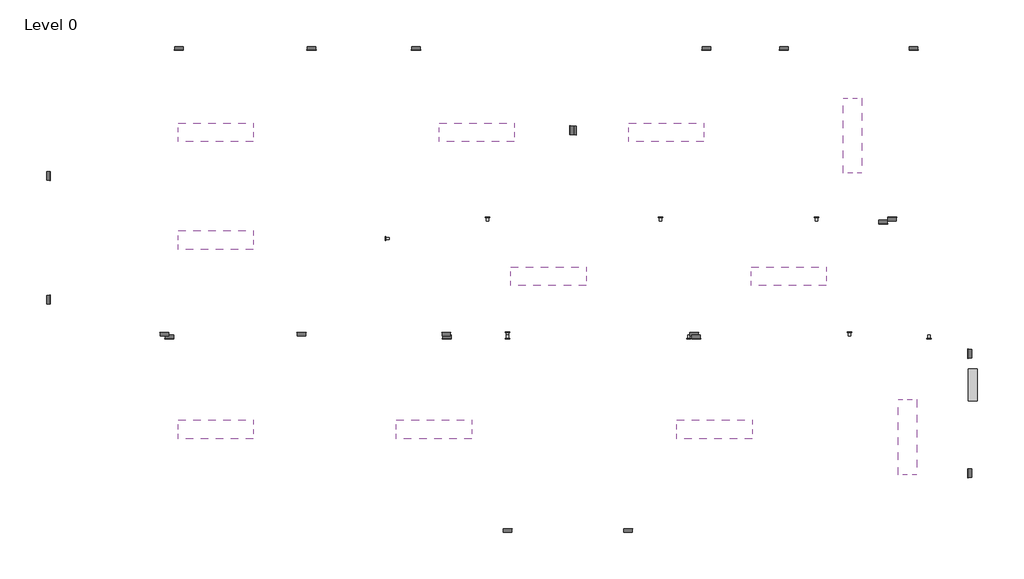
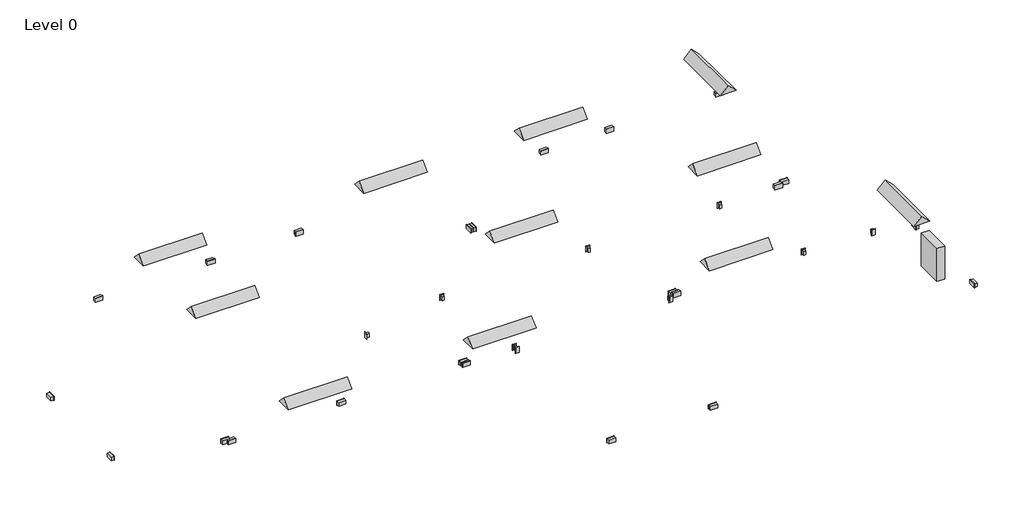
# One storey: 24 proxies, 11 light fixtures, 9 switching devices.
"""IFC4 building model written with IfcOpenShell, lengths in millimetres."""

import ifcopenshell
import ifcopenshell.guid

model = None  # the IFC model being written
_history = None  # IfcOwnerHistory: only IFC2X3 demands one
_inside = {}  # id of a spatial element -> (the spatial element, [elements in it])
_under = {}  # id of a project, library or spatial element -> (it, [spatial elements below it])
_declared = {}  # id of a project -> (the project, [libraries it declares])
_typed = {}  # id of a type object -> (the type object, [elements of that type])
_made_of = {}  # id of a material, layer set ... -> (it, [elements and type objects made of it])


def new_model(schema):
    """Start an empty IFC model of exactly this schema.

    Asked for "IFC4X3", IfcOpenShell would pick the latest addendum, in which some entities
    have other attributes; the version numbers below select the first issue.
    IFC2X3 requires an IfcOwnerHistory on every rooted entity: one is made here for all.
    """
    global model, _history
    if schema == "IFC4X3":
        model = ifcopenshell.file(schema_version=(4, 3, 0, 0))
    else:
        model = ifcopenshell.file(schema=schema)
    _inside.clear()
    _under.clear()
    _declared.clear()
    _typed.clear()
    _made_of.clear()
    _history = None
    if model.schema == "IFC2X3":
        org = make("IfcOrganization", Name="unknown")
        user = make(
            "IfcPersonAndOrganization",
            ThePerson=make("IfcPerson", FamilyName="unknown"),
            TheOrganization=org,
        )
        app = make(
            "IfcApplication",
            ApplicationDeveloper=org,
            Version="unknown",
            ApplicationFullName="unknown",
            ApplicationIdentifier="unknown",
        )
        _history = make(
            "IfcOwnerHistory",
            OwningUser=user,
            OwningApplication=app,
            ChangeAction="ADDED",
            CreationDate=0,
        )
    return model


def make(cls, **values):
    """One entity of the class cls with the attributes given. An attribute that is None is left unset."""
    return model.create_entity(
        cls, **{name: value for name, value in values.items() if value is not None}
    )


def rooted(cls, **values):
    """An entity with a GlobalId (a new one), such as an element, a storey or a relation."""
    return make(cls, GlobalId=ifcopenshell.guid.new(), OwnerHistory=_history, **values)


def si_unit(unit_type, name, prefix=None):
    """IfcSIUnit, for example si_unit("LENGTHUNIT", "METRE", prefix="MILLI")."""
    return make("IfcSIUnit", UnitType=unit_type, Prefix=prefix, Name=name)


def assignment(units):
    """IfcUnitAssignment: the units of a project."""
    return None if units is None else make("IfcUnitAssignment", Units=units)


def point(xyz):
    """IfcCartesianPoint."""
    return None if xyz is None else make("IfcCartesianPoint", Coordinates=xyz)


def direction(xyz):
    """IfcDirection."""
    return None if xyz is None else make("IfcDirection", DirectionRatios=xyz)


def frame(location, z_axis=None, x_axis=None):
    """IfcAxis2Placement3D, a coordinate frame: its origin and axes. An axis left out is left unset."""
    return make(
        "IfcAxis2Placement3D",
        Location=point(location),
        Axis=direction(z_axis),
        RefDirection=direction(x_axis),
    )


def origin():
    """The frame at (0, 0, 0) with its axes left unset."""
    return frame((0.0, 0.0, 0.0))


def origin_with_axes():
    """The frame at (0, 0, 0) with the z axis (0, 0, 1) and the x axis (1, 0, 0) written out."""
    return frame((0.0, 0.0, 0.0), z_axis=(0.0, 0.0, 1.0), x_axis=(1.0, 0.0, 0.0))


def place(relative_to, where):
    """IfcLocalPlacement: puts the frame where relative to a parent placement (None: the world)."""
    return make(
        "IfcLocalPlacement", PlacementRelTo=relative_to, RelativePlacement=where
    )


def context(
    kind, dimensions, precision=None, world=None, true_north=None, identifier=None
):
    """IfcGeometricRepresentationContext, for example the 3D "Model" context."""
    return make(
        "IfcGeometricRepresentationContext",
        ContextIdentifier=identifier,
        ContextType=kind,
        CoordinateSpaceDimension=dimensions,
        Precision=precision,
        WorldCoordinateSystem=world,
        TrueNorth=true_north,
    )


def project(units=None, contexts=None):
    """IfcProject with its units and contexts."""
    return rooted(
        "IfcProject",
        Name="project",
        RepresentationContexts=contexts,
        UnitsInContext=assignment(units),
    )


def spatial(cls, under=None, at=None, **own):
    """A site, building, storey or space (cls), placed at a placement, below another one or the project."""
    s = rooted(cls, ObjectPlacement=at, **own)
    if under is not None:
        _under.setdefault(under.id(), (under, []))[1].append(s)
    return s


def polyline(points):
    """IfcPolyline through the points."""
    return make("IfcPolyline", Points=[point(p) for p in points])


def outline(outer, holes=None, kind="AREA"):
    """IfcArbitraryClosedProfileDef: a profile drawn as a closed curve; with holes, ...WithVoids."""
    if holes is None:
        return make("IfcArbitraryClosedProfileDef", ProfileType=kind, OuterCurve=outer)
    return make(
        "IfcArbitraryProfileDefWithVoids",
        ProfileType=kind,
        OuterCurve=outer,
        InnerCurves=holes,
    )


def extrude(swept, where, along, depth):
    """IfcExtrudedAreaSolid: the profile swept, set in the frame where, extruded along a direction by depth."""
    return make(
        "IfcExtrudedAreaSolid",
        SweptArea=swept,
        Position=where,
        ExtrudedDirection=direction(along),
        Depth=depth,
    )


def shape(context_of_items, identifier, shape_type, items):
    """IfcShapeRepresentation: the items that make up one representation, for example the "Body"."""
    return make(
        "IfcShapeRepresentation",
        ContextOfItems=context_of_items,
        RepresentationIdentifier=identifier,
        RepresentationType=shape_type,
        Items=items,
    )


def source(mapping_origin, context_of_items, identifier, shape_type, items):
    """IfcRepresentationMap: a shape defined once, which mapped items show again and again."""
    return make(
        "IfcRepresentationMap",
        MappingOrigin=mapping_origin,
        MappedRepresentation=shape(context_of_items, identifier, shape_type, items),
    )


def transform(
    local_origin,
    x_axis=None,
    y_axis=None,
    z_axis=None,
    scale=None,
    scale2=None,
    scale3=None,
    uniform=True,
):
    """IfcCartesianTransformationOperator3D, or its non-uniform kind. x_axis, y_axis, z_axis: its Axis1, 2, 3."""
    if uniform:
        return make(
            "IfcCartesianTransformationOperator3D",
            Axis1=direction(x_axis),
            Axis2=direction(y_axis),
            LocalOrigin=point(local_origin),
            Scale=scale,
            Axis3=direction(z_axis),
        )
    return make(
        "IfcCartesianTransformationOperator3DnonUniform",
        Axis1=direction(x_axis),
        Axis2=direction(y_axis),
        LocalOrigin=point(local_origin),
        Scale=scale,
        Axis3=direction(z_axis),
        Scale2=scale2,
        Scale3=scale3,
    )


def mapped(mapping_source, mapping_target):
    """IfcMappedItem: shows the shape of a source again, moved by a transform."""
    return make(
        "IfcMappedItem", MappingSource=mapping_source, MappingTarget=mapping_target
    )


def made_of(thing, what):
    """Note that an element or type object is made of a material, layer set ...; save() writes the relation."""
    if what is not None:
        _made_of.setdefault(what.id(), (what, []))[1].append(thing)
    return thing


def element(
    cls,
    number,
    at=None,
    inside=None,
    cuts=None,
    type_object=None,
    material=None,
    context=None,
    identifier="Body",
    shape_type=None,
    held_by="IfcProductDefinitionShape",
    body=None,
    shapes=None,
    **own,
):
    """One element of the class cls, such as IfcWall. Its Tag is "e" and its number.

    at: its placement. inside: the storey or other place that contains it. cuts: it is an
    opening in that element (IfcRelVoidsElement). A single representation is given by context,
    identifier, shape_type and body (its items); several are given by shapes. held_by: the class
    of the entity that holds the representations. save() writes the other relations.
    """
    e = rooted(cls, Tag="e%d" % number, ObjectPlacement=at, **own)
    if body is not None:
        shapes = [shape(context, identifier, shape_type, body)]
    if shapes is not None:
        e.Representation = make(held_by, Representations=shapes)
    if inside is not None:
        _inside.setdefault(inside.id(), (inside, []))[1].append(e)
    if cuts is not None:
        rooted(
            "IfcRelVoidsElement", RelatingBuildingElement=cuts, RelatedOpeningElement=e
        )
    if type_object is not None:
        _typed.setdefault(type_object.id(), (type_object, []))[1].append(e)
    return made_of(e, material)


def aggregate(whole, parts):
    """IfcRelAggregates: a whole, such as a stair, and the parts it consists of."""
    return rooted("IfcRelAggregates", RelatingObject=whole, RelatedObjects=parts)


def save(model, path):
    """Write the relations noted so far, then the file.

    IfcRelAggregates (storeys below a building ...), IfcRelContainedInSpatialStructure (elements
    in a storey), IfcRelDefinesByType, IfcRelAssociatesMaterial and IfcRelDeclares: one each for
    every whole, place, type object, material and project.
    """
    for whole, parts in _under.values():
        aggregate(whole, parts)
    for where, things in _inside.values():
        rooted(
            "IfcRelContainedInSpatialStructure",
            RelatedElements=things,
            RelatingStructure=where,
        )
    for kind, things in _typed.values():
        rooted("IfcRelDefinesByType", RelatedObjects=things, RelatingType=kind)
    for what, things in _made_of.values():
        rooted("IfcRelAssociatesMaterial", RelatedObjects=things, RelatingMaterial=what)
    for by, libraries in _declared.values():
        rooted("IfcRelDeclares", RelatingContext=by, RelatedDefinitions=libraries)
    model.write(path)


def lighting_and_appliance_panelboard_400v_mlo_125_a_11cb7106(model_context):
    return source(origin(), model_context, "Body", "SweptSolid", [
        extrude(outline(polyline([(254.0, -660.4), (-254.0, -660.4), (-254.0, 0.0), (254.0, 0.0), (254.0, -660.4)])), frame((0.0, 0.0, -146.1), z_axis=(0.0, 0.0, 1.0), x_axis=(1.0, 0.0, 0.0)), (0.0, 0.0, 1.0), 146.1),
    ])


def twin_switched_socket_outlet_standard_0deee84c(model_context):
    return source(origin(), model_context, "Body", "SweptSolid", [
        extrude(outline(polyline([(67.5, 37.5), (67.5, -37.5), (-67.5, -37.5), (-67.5, 37.5), (67.5, 37.5)])), frame((0.0, 0.0, -53.975), z_axis=(0.0, 0.0, 1.0), x_axis=(1.0, 0.0, 0.0)), (0.0, 0.0, 1.0), 53.975),
        extrude(outline(polyline([(72.5, 42.5), (72.5, -42.5), (-72.5, -42.5), (-72.5, 42.5), (72.5, 42.5)])), origin_with_axes(), (0.0, 0.0, 1.0), 4.7625),
    ])


def plain_recessed_lighting_fixture_300x1200_230_e46e8774(model_context):
    return source(origin(), model_context, "Body", "SweptSolid", [
        extrude(outline(polyline([(-300.0, 0.0), (0.0, 0.0), (-150.0, -150.0), (-300.0, 0.0)])), frame((0.0, 0.0, 0.0), z_axis=(1.0, 0.0, 0.0), x_axis=(0.0, 1.0, 0.0)), (0.0, 0.0, 1.0), 1200.0),
    ])


def lighting_switches_one_way_switch_9cbd35ee(model_context):
    return source(origin(), model_context, "Body", "SweptSolid", [
        extrude(outline(polyline([(35.0, -114.0), (-35.0, -114.0), (-35.0, 0.0), (35.0, 0.0), (35.0, -114.0)])), origin_with_axes(), (0.0, 0.0, 1.0), 5.0),
        extrude(outline(polyline([(19.0, -95.0), (-19.0, -95.0), (-19.0, -19.0), (19.0, -19.0), (19.0, -95.0)])), frame((0.0, 0.0, -54.0), z_axis=(0.0, 0.0, 1.0), x_axis=(1.0, 0.0, 0.0)), (0.0, 0.0, 1.0), 54.0),
    ])


model = new_model("IFC4")

# Units and contexts
model_context = context("Model", 3, world=origin())
ifc_project = project(units=[si_unit("LENGTHUNIT", "METRE", prefix="MILLI")], contexts=[model_context])

# Site, building, storey
site = spatial("IfcSite", under=ifc_project)
building = spatial("IfcBuilding", under=site)
storey = spatial("IfcBuildingStorey", under=building, Name="Level 0", Elevation=0.0)

# Proxies
placement = place(None, origin())
lighting_and_appliance_panelboard_400v_mlo_125_a_shape = lighting_and_appliance_panelboard_400v_mlo_125_a_11cb7106(model_context)
element("IfcBuildingElementProxy", 1, Name="Lighting and Appliance Panelboard - 400V MLO : 125 A", ObjectType="Lighting and Appliance Panelboard - 400V MLO : 125 A", at=placement, inside=storey, context=model_context, shape_type="MappedRepresentation", body=[
    mapped(lighting_and_appliance_panelboard_400v_mlo_125_a_shape, transform((7333.0126521, -1228.5996446, 1200.0), x_axis=(0.0, -1.0, 0.0), y_axis=(0.0, 0.0, 1.0), z_axis=(-1.0, 0.0, 0.0))),
])
twin_switched_socket_outlet_standard_shape = twin_switched_socket_outlet_standard_0deee84c(model_context)
element("IfcBuildingElementProxy", 2, Name="Twin Switched Socket Outlet : Standard", ObjectType="Twin Switched Socket Outlet : Standard", at=placement, inside=storey, context=model_context, shape_type="MappedRepresentation", body=[
    mapped(twin_switched_socket_outlet_standard_shape, transform((7333.0126521, -731.9030192, 1200.0), x_axis=(0.0, -1.0, 0.0), y_axis=(0.0, 0.0, 1.0), z_axis=(-1.0, 0.0, 0.0))),
])
element("IfcBuildingElementProxy", 3, Name="Twin Switched Socket Outlet : Standard", ObjectType="Twin Switched Socket Outlet : Standard", at=placement, inside=storey, context=model_context, shape_type="MappedRepresentation", body=[
    mapped(twin_switched_socket_outlet_standard_shape, transform((7333.0126521, -2640.7763248, 1200.0), x_axis=(0.0, -1.0, 0.0), y_axis=(0.0, 0.0, 1.0), z_axis=(-1.0, 0.0, 0.0))),
])
element("IfcBuildingElementProxy", 4, Name="Twin Switched Socket Outlet : Standard", ObjectType="Twin Switched Socket Outlet : Standard", at=placement, inside=storey, context=model_context, shape_type="MappedRepresentation", body=[
    mapped(twin_switched_socket_outlet_standard_shape, transform((1908.0707872, -3530.9314954, 1200.0), x_axis=(-1.0, 0.0, 0.0), y_axis=(0.0, 0.0, 1.0), z_axis=(0.0, 1.0, 0.0))),
])
element("IfcBuildingElementProxy", 5, Name="Twin Switched Socket Outlet : Standard", ObjectType="Twin Switched Socket Outlet : Standard", at=placement, inside=storey, context=model_context, shape_type="MappedRepresentation", body=[
    mapped(twin_switched_socket_outlet_standard_shape, transform((2992.0804727, -488.4314954, 1200.0), x_axis=(1.0, 0.0, 0.0), y_axis=(0.0, 0.0, 1.0), z_axis=(0.0, -1.0, 0.0))),
])
element("IfcBuildingElementProxy", 6, Name="Twin Switched Socket Outlet : Standard", ObjectType="Twin Switched Socket Outlet : Standard", at=placement, inside=storey, context=model_context, shape_type="MappedRepresentation", body=[
    mapped(twin_switched_socket_outlet_standard_shape, transform((2958.20517, -393.4314954, 1200.0), x_axis=(-1.0, 0.0, 0.0), y_axis=(0.0, 0.0, 1.0), z_axis=(0.0, 1.0, 0.0))),
])
element("IfcBuildingElementProxy", 7, Name="Twin Switched Socket Outlet : Standard", ObjectType="Twin Switched Socket Outlet : Standard", at=placement, inside=storey, context=model_context, shape_type="MappedRepresentation", body=[
    mapped(twin_switched_socket_outlet_standard_shape, transform((-14.3526395, -3530.9314954, 1200.0), x_axis=(-1.0, 0.0, 0.0), y_axis=(0.0, 0.0, 1.0), z_axis=(0.0, 1.0, 0.0))),
])
element("IfcBuildingElementProxy", 8, Name="Twin Switched Socket Outlet : Standard", ObjectType="Twin Switched Socket Outlet : Standard", at=placement, inside=storey, context=model_context, shape_type="MappedRepresentation", body=[
    mapped(twin_switched_socket_outlet_standard_shape, transform((4391.3814995, 4119.0685046, 1200.0), x_axis=(1.0, 0.0, 0.0), y_axis=(0.0, 0.0, 1.0), z_axis=(0.0, -1.0, 0.0))),
])
element("IfcBuildingElementProxy", 9, Name="Twin Switched Socket Outlet : Standard", ObjectType="Twin Switched Socket Outlet : Standard", at=placement, inside=storey, context=model_context, shape_type="MappedRepresentation", body=[
    mapped(twin_switched_socket_outlet_standard_shape, transform((6460.720641, 4119.0685046, 1200.0), x_axis=(1.0, 0.0, 0.0), y_axis=(0.0, 0.0, 1.0), z_axis=(0.0, -1.0, 0.0))),
])
element("IfcBuildingElementProxy", 10, Name="Twin Switched Socket Outlet : Standard", ObjectType="Twin Switched Socket Outlet : Standard", at=placement, inside=storey, context=model_context, shape_type="MappedRepresentation", body=[
    mapped(twin_switched_socket_outlet_standard_shape, transform((3154.1965323, 4119.0685046, 1200.0), x_axis=(1.0, 0.0, 0.0), y_axis=(0.0, 0.0, 1.0), z_axis=(0.0, -1.0, 0.0))),
])
element("IfcBuildingElementProxy", 11, Name="Twin Switched Socket Outlet : Standard", ObjectType="Twin Switched Socket Outlet : Standard", at=placement, inside=storey, context=model_context, shape_type="MappedRepresentation", body=[
    mapped(twin_switched_socket_outlet_standard_shape, transform((-1477.8828984, 4119.0685046, 1200.0), x_axis=(1.0, 0.0, 0.0), y_axis=(0.0, 0.0, 1.0), z_axis=(0.0, -1.0, 0.0))),
])
element("IfcBuildingElementProxy", 12, Name="Twin Switched Socket Outlet : Standard", ObjectType="Twin Switched Socket Outlet : Standard", at=placement, inside=storey, context=model_context, shape_type="MappedRepresentation", body=[
    mapped(twin_switched_socket_outlet_standard_shape, transform((-994.5789843, -393.4314954, 1200.0), x_axis=(-1.0, 0.0, 0.0), y_axis=(0.0, 0.0, 1.0), z_axis=(0.0, 1.0, 0.0))),
])
element("IfcBuildingElementProxy", 13, Name="Twin Switched Socket Outlet : Standard", ObjectType="Twin Switched Socket Outlet : Standard", at=placement, inside=storey, context=model_context, shape_type="MappedRepresentation", body=[
    mapped(twin_switched_socket_outlet_standard_shape, transform((-983.8752261, -488.4314954, 1200.0), x_axis=(1.0, 0.0, 0.0), y_axis=(0.0, 0.0, 1.0), z_axis=(0.0, -1.0, 0.0))),
])
element("IfcBuildingElementProxy", 14, Name="Twin Switched Socket Outlet : Standard", ObjectType="Twin Switched Socket Outlet : Standard", at=placement, inside=storey, context=model_context, shape_type="MappedRepresentation", body=[
    mapped(twin_switched_socket_outlet_standard_shape, transform((-7316.9873479, 2106.2473929, 1200.0), x_axis=(0.0, 1.0, 0.0), y_axis=(0.0, 0.0, 1.0), z_axis=(1.0, 0.0, 0.0))),
])
element("IfcBuildingElementProxy", 15, Name="Twin Switched Socket Outlet : Standard", ObjectType="Twin Switched Socket Outlet : Standard", at=placement, inside=storey, context=model_context, shape_type="MappedRepresentation", body=[
    mapped(twin_switched_socket_outlet_standard_shape, transform((-7316.9873479, 133.0110122, 1200.0), x_axis=(0.0, 1.0, 0.0), y_axis=(0.0, 0.0, 1.0), z_axis=(1.0, 0.0, 0.0))),
])
element("IfcBuildingElementProxy", 16, Name="Twin Switched Socket Outlet : Standard", ObjectType="Twin Switched Socket Outlet : Standard", at=placement, inside=storey, context=model_context, shape_type="MappedRepresentation", body=[
    mapped(twin_switched_socket_outlet_standard_shape, transform((-5491.7999145, -393.4314954, 1200.0), x_axis=(-1.0, 0.0, 0.0), y_axis=(0.0, 0.0, 1.0), z_axis=(0.0, 1.0, 0.0))),
])
element("IfcBuildingElementProxy", 17, Name="Twin Switched Socket Outlet : Standard", ObjectType="Twin Switched Socket Outlet : Standard", at=placement, inside=storey, context=model_context, shape_type="MappedRepresentation", body=[
    mapped(twin_switched_socket_outlet_standard_shape, transform((-5410.6999104, -488.4314954, 1200.0), x_axis=(1.0, 0.0, 0.0), y_axis=(0.0, 0.0, 1.0), z_axis=(0.0, -1.0, 0.0))),
])
element("IfcBuildingElementProxy", 18, Name="Twin Switched Socket Outlet : Standard", ObjectType="Twin Switched Socket Outlet : Standard", at=placement, inside=storey, context=model_context, shape_type="MappedRepresentation", body=[
    mapped(twin_switched_socket_outlet_standard_shape, transform((-5260.1397144, 4119.0685046, 1200.0), x_axis=(1.0, 0.0, 0.0), y_axis=(0.0, 0.0, 1.0), z_axis=(0.0, -1.0, 0.0))),
])
element("IfcBuildingElementProxy", 19, Name="Twin Switched Socket Outlet : Standard", ObjectType="Twin Switched Socket Outlet : Standard", at=placement, inside=storey, context=model_context, shape_type="MappedRepresentation", body=[
    mapped(twin_switched_socket_outlet_standard_shape, transform((-3144.1513827, 4119.0685046, 1200.0), x_axis=(1.0, 0.0, 0.0), y_axis=(0.0, 0.0, 1.0), z_axis=(0.0, -1.0, 0.0))),
])
element("IfcBuildingElementProxy", 20, Name="Twin Switched Socket Outlet : Standard", ObjectType="Twin Switched Socket Outlet : Standard", at=placement, inside=storey, context=model_context, shape_type="MappedRepresentation", body=[
    mapped(twin_switched_socket_outlet_standard_shape, transform((-3304.0957389, -393.4314954, 1200.0), x_axis=(-1.0, 0.0, 0.0), y_axis=(0.0, 0.0, 1.0), z_axis=(0.0, 1.0, 0.0))),
])
element("IfcBuildingElementProxy", 21, Name="Twin Switched Socket Outlet : Standard", ObjectType="Twin Switched Socket Outlet : Standard", at=placement, inside=storey, context=model_context, shape_type="MappedRepresentation", body=[
    mapped(twin_switched_socket_outlet_standard_shape, transform((983.0126521, 2835.1015679, 1200.0), x_axis=(0.0, -1.0, 0.0), y_axis=(0.0, 0.0, 1.0), z_axis=(-1.0, 0.0, 0.0))),
])
element("IfcBuildingElementProxy", 22, Name="Twin Switched Socket Outlet : Standard", ObjectType="Twin Switched Socket Outlet : Standard", at=placement, inside=storey, context=model_context, shape_type="MappedRepresentation", body=[
    mapped(twin_switched_socket_outlet_standard_shape, transform((1078.0126521, 2831.4402609, 1200.0), x_axis=(0.0, 1.0, 0.0), y_axis=(0.0, 0.0, 1.0), z_axis=(1.0, 0.0, 0.0))),
])
element("IfcBuildingElementProxy", 23, Name="Twin Switched Socket Outlet : Standard", ObjectType="Twin Switched Socket Outlet : Standard", at=placement, inside=storey, context=model_context, shape_type="MappedRepresentation", body=[
    mapped(twin_switched_socket_outlet_standard_shape, transform((5974.113816, 1346.5685046, 1200.0), x_axis=(1.0, 0.0, 0.0), y_axis=(0.0, 0.0, 1.0), z_axis=(0.0, -1.0, 0.0))),
])
element("IfcBuildingElementProxy", 24, Name="Twin Switched Socket Outlet : Standard", ObjectType="Twin Switched Socket Outlet : Standard", at=placement, inside=storey, context=model_context, shape_type="MappedRepresentation", body=[
    mapped(twin_switched_socket_outlet_standard_shape, transform((6119.3761729, 1441.5685046, 1200.0), x_axis=(-1.0, 0.0, 0.0), y_axis=(0.0, 0.0, 1.0), z_axis=(0.0, 1.0, 0.0))),
])

# Light fixtures
plain_recessed_lighting_fixture_300x1200_230_shape = plain_recessed_lighting_fixture_300x1200_230_e46e8774(model_context)
element("IfcLightFixture", 25, ObjectType="Plain Recessed Lighting Fixture : 300x1200 - 230", at=placement, inside=storey, context=model_context, shape_type="MappedRepresentation", body=[
    mapped(plain_recessed_lighting_fixture_300x1200_230_shape, transform((-5270.0307392, 2652.1798309, 2750.0), x_axis=(1.0, 0.0, 0.0), y_axis=(0.0, -1.0, 0.0), z_axis=(0.0, 0.0, -1.0))),
])
element("IfcLightFixture", 26, ObjectType="Plain Recessed Lighting Fixture : 300x1200 - 230", at=placement, inside=storey, context=model_context, shape_type="MappedRepresentation", body=[
    mapped(plain_recessed_lighting_fixture_300x1200_230_shape, transform((-5270.0307392, 932.4806964, 2750.0), x_axis=(1.0, 0.0, 0.0), y_axis=(0.0, -1.0, 0.0), z_axis=(0.0, 0.0, -1.0))),
])
element("IfcLightFixture", 27, ObjectType="Plain Recessed Lighting Fixture : 300x1200 - 230", at=placement, inside=storey, context=model_context, shape_type="MappedRepresentation", body=[
    mapped(plain_recessed_lighting_fixture_300x1200_230_shape, transform((-5270.0307392, -2089.1732245, 2750.0), x_axis=(1.0, 0.0, 0.0), y_axis=(0.0, -1.0, 0.0), z_axis=(0.0, 0.0, -1.0))),
])
element("IfcLightFixture", 28, ObjectType="Plain Recessed Lighting Fixture : 300x1200 - 230", at=placement, inside=storey, context=model_context, shape_type="MappedRepresentation", body=[
    mapped(plain_recessed_lighting_fixture_300x1200_230_shape, transform((-1789.2039186, -2089.1732245, 2750.0), x_axis=(1.0, 0.0, 0.0), y_axis=(0.0, -1.0, 0.0), z_axis=(0.0, 0.0, -1.0))),
])
element("IfcLightFixture", 29, ObjectType="Plain Recessed Lighting Fixture : 300x1200 - 230", at=placement, inside=storey, context=model_context, shape_type="MappedRepresentation", body=[
    mapped(plain_recessed_lighting_fixture_300x1200_230_shape, transform((2684.0288466, -2089.1732245, 2750.0), x_axis=(1.0, 0.0, 0.0), y_axis=(0.0, -1.0, 0.0), z_axis=(0.0, 0.0, -1.0))),
])
element("IfcLightFixture", 30, ObjectType="Plain Recessed Lighting Fixture : 300x1200 - 230", at=placement, inside=storey, context=model_context, shape_type="MappedRepresentation", body=[
    mapped(plain_recessed_lighting_fixture_300x1200_230_shape, transform((-1107.8505835, 2652.1798309, 2750.0), x_axis=(1.0, 0.0, 0.0), y_axis=(0.0, -1.0, 0.0), z_axis=(0.0, 0.0, -1.0))),
])
element("IfcLightFixture", 31, ObjectType="Plain Recessed Lighting Fixture : 300x1200 - 230", at=placement, inside=storey, context=model_context, shape_type="MappedRepresentation", body=[
    mapped(plain_recessed_lighting_fixture_300x1200_230_shape, transform((1913.8033373, 2652.1798309, 2750.0), x_axis=(1.0, 0.0, 0.0), y_axis=(0.0, -1.0, 0.0), z_axis=(0.0, 0.0, -1.0))),
])
element("IfcLightFixture", 32, ObjectType="Plain Recessed Lighting Fixture : 300x1200 - 230", at=placement, inside=storey, context=model_context, shape_type="MappedRepresentation", body=[
    mapped(plain_recessed_lighting_fixture_300x1200_230_shape, transform((5336.1226433, 3350.5669994, 2750.0), x_axis=(0.0, -1.0, 0.0), y_axis=(-1.0, 0.0, 0.0), z_axis=(0.0, 0.0, -1.0))),
])
element("IfcLightFixture", 33, ObjectType="Plain Recessed Lighting Fixture : 300x1200 - 230", at=placement, inside=storey, context=model_context, shape_type="MappedRepresentation", body=[
    mapped(plain_recessed_lighting_fixture_300x1200_230_shape, transform((35.7584033, 354.8115644, 2750.0), x_axis=(1.0, 0.0, 0.0), y_axis=(0.0, -1.0, 0.0), z_axis=(0.0, 0.0, -1.0))),
])
element("IfcLightFixture", 34, ObjectType="Plain Recessed Lighting Fixture : 300x1200 - 230", at=placement, inside=storey, context=model_context, shape_type="MappedRepresentation", body=[
    mapped(plain_recessed_lighting_fixture_300x1200_230_shape, transform((3868.9911685, 354.8115644, 2750.0), x_axis=(1.0, 0.0, 0.0), y_axis=(0.0, -1.0, 0.0), z_axis=(0.0, 0.0, -1.0))),
])
element("IfcLightFixture", 35, ObjectType="Plain Recessed Lighting Fixture : 300x1200 - 230", at=placement, inside=storey, context=model_context, shape_type="MappedRepresentation", body=[
    mapped(plain_recessed_lighting_fixture_300x1200_230_shape, transform((6212.25416, -1465.5868026, 2750.0), x_axis=(0.0, -1.0, 0.0), y_axis=(-1.0, 0.0, 0.0), z_axis=(0.0, 0.0, -1.0))),
])

# Switching devices
lighting_switches_one_way_switch_shape = lighting_switches_one_way_switch_9cbd35ee(model_context)
element("IfcSwitchingDevice", 36, ObjectType="Lighting Switches : One Way Switch", at=placement, inside=storey, context=model_context, shape_type="MappedRepresentation", body=[
    mapped(lighting_switches_one_way_switch_shape, transform((-1959.4873479, 1106.2790704, 1200.0), x_axis=(0.0, -1.0, 0.0), y_axis=(0.0, 0.0, 1.0), z_axis=(-1.0, 0.0, 0.0))),
])
element("IfcSwitchingDevice", 37, ObjectType="Lighting Switches : One Way Switch", at=placement, inside=storey, context=model_context, shape_type="MappedRepresentation", body=[
    mapped(lighting_switches_one_way_switch_shape, transform((-334.0931611, 1441.5685046, 1200.0), x_axis=(-1.0, 0.0, 0.0), y_axis=(0.0, 0.0, 1.0), z_axis=(0.0, 1.0, 0.0))),
])
element("IfcSwitchingDevice", 38, ObjectType="Lighting Switches : One Way Switch", at=placement, inside=storey, context=model_context, shape_type="MappedRepresentation", body=[
    mapped(lighting_switches_one_way_switch_shape, transform((2425.9086107, 1441.5685046, 1200.0), x_axis=(-1.0, 0.0, 0.0), y_axis=(0.0, 0.0, 1.0), z_axis=(0.0, 1.0, 0.0))),
])
element("IfcSwitchingDevice", 39, ObjectType="Lighting Switches : One Way Switch", at=placement, inside=storey, context=model_context, shape_type="MappedRepresentation", body=[
    mapped(lighting_switches_one_way_switch_shape, transform((4910.5243833, 1441.5685046, 1200.0), x_axis=(-1.0, 0.0, 0.0), y_axis=(0.0, 0.0, 1.0), z_axis=(0.0, 1.0, 0.0))),
])
element("IfcSwitchingDevice", 40, ObjectType="Lighting Switches : One Way Switch", at=placement, inside=storey, context=model_context, shape_type="MappedRepresentation", body=[
    mapped(lighting_switches_one_way_switch_shape, transform((6703.5460749, -488.4314954, 1200.0), x_axis=(1.0, 0.0, 0.0), y_axis=(0.0, 0.0, 1.0), z_axis=(0.0, -1.0, 0.0))),
])
element("IfcSwitchingDevice", 41, ObjectType="Lighting Switches : One Way Switch", at=placement, inside=storey, context=model_context, shape_type="MappedRepresentation", body=[
    mapped(lighting_switches_one_way_switch_shape, transform((2874.1640336, -488.4314954, 1200.0), x_axis=(1.0, 0.0, 0.0), y_axis=(0.0, 0.0, 1.0), z_axis=(0.0, -1.0, 0.0))),
])
element("IfcSwitchingDevice", 42, ObjectType="Lighting Switches : One Way Switch", at=placement, inside=storey, context=model_context, shape_type="MappedRepresentation", body=[
    mapped(lighting_switches_one_way_switch_shape, transform((-20.2852685, -488.4314954, 1200.0), x_axis=(1.0, 0.0, 0.0), y_axis=(0.0, 0.0, 1.0), z_axis=(0.0, -1.0, 0.0))),
])
element("IfcSwitchingDevice", 43, ObjectType="Lighting Switches : Two Way Switch", at=placement, inside=storey, context=model_context, shape_type="MappedRepresentation", body=[
    mapped(lighting_switches_one_way_switch_shape, transform((-18.1392133, -393.4314954, 1200.0), x_axis=(-1.0, 0.0, 0.0), y_axis=(0.0, 0.0, 1.0), z_axis=(0.0, 1.0, 0.0))),
])
element("IfcSwitchingDevice", 44, ObjectType="Lighting Switches : Two Way Switch", at=placement, inside=storey, context=model_context, shape_type="MappedRepresentation", body=[
    mapped(lighting_switches_one_way_switch_shape, transform((5435.784517, -393.4314954, 1200.0), x_axis=(-1.0, 0.0, 0.0), y_axis=(0.0, 0.0, 1.0), z_axis=(0.0, 1.0, 0.0))),
])

save(model, "model.ifc")

# Revit data of these elements
# Project information
#   Project Issue Date = "Oct 2020"
#   Project Status = "Project Status"
#   Client Name = "Your Name Here"
#   Project Address = "Enter address here"
#   Project Name = "Revit MEP 01"
#   Project Number = "RMEP01"
# Type "Lighting and Appliance Panelboard - 400V MLO : 125 A"
#   built-in parameter 1140081 [instance default] = "Recessed"
#   built-in parameter 1140083 [instance default] = "Type 1"
#   Width = 508 mm
#   built-in parameter 1140082 [instance default] = 100 (stored number, unit not read)
#   built-in parameter 1140140 [instance default] = 1 (stored number, unit not read)
#   Height [instance default] = 660.4 mm
#   Depth = 146.1 mm
#   Default Elevation = 1200 mm
#   42 Circuit Height = 1117.6 mm
#   30 Circuit Height = 965.2 mm
#   18 Circuit Height = 660.4 mm
#   12 Circuit Height = 660.4 mm
#   built-in parameter 1140142 [instance default] = -1
#   built-in parameter 1140079 [instance default] = 12
#   built-in parameter 1155100 [instance default] = -1
#   Load Classification = Other
#   built-in parameter 1140087 [instance default] = element -7000014
# Type "Twin Switched Socket Outlet : Standard"
#   Label = "2"
#   Switch Voltage = 230 V
#   Load = 180 VA
#   Default Elevation = 1200 mm
#   Load Classification = Socket
#   Assembly Code = ""
# Type "Plain Recessed Lighting Fixture : 300x1200 - 230"
#   Photometric Web File = "1x42A12.ies"
#   Width = 300 mm
#   Wattage = 64 W
#   built-in parameter 1150110 = 1 (stored number, unit not read)
#   built-in parameter 1150109 = 1 (stored number, unit not read)
#   built-in parameter 1150113 = 1 (stored number, unit not read)
#   Tilt Angle = -90.00°
#   Lumens = 5699.84 lm
#   built-in parameter 1114217 = 0.88 (stored number, unit not read)
#   built-in parameter 1150115 = 1 (stored number, unit not read)
#   built-in parameter 1150105 = 453.579 (stored number, unit not read)
#   Length = 1200 mm
#   built-in parameter 1150112 = 1 (stored number, unit not read)
#   built-in parameter 1150114 = 1 (stored number, unit not read)
#   built-in parameter 1150107 = 4230 (stored number, unit not read)
#   built-in parameter 1150106 = 4.53579 (stored number, unit not read)
#   Emit from Rectangle Width = 300 mm
#   Emit from Rectangle Length = 1200 mm
#   built-in parameter 1150104 = 8.27394 (stored number, unit not read)
#   Depth = 150 mm
#   Default Elevation = 2000 mm
#   Ballast Voltage = 230 V
#   built-in parameter 1114218 = 0.88 (stored number, unit not read)
#   built-in parameter 1150133 = 10 (stored number, unit not read)
#   Apparent Load = 64 VA
#   built-in parameter 1150134 = 8
#   built-in parameter 1150137 = 1
#   Color Filter = 16777215
#   built-in parameter 1140040 [instance default] = 1
#   Load Classification = Lighting - Dwelling Unit
#   Emit Shape Visible in Rendering = no
#   Dimming Lamp Color Temperature Shift = (empty or 0)
#   Assembly Code = ""
# Type "Lighting Switches : One Way Switch"
#   Label = ""
#   Width = 70 mm
#   Switch Voltage [instance default] = 230 V
#   Length = 114 mm
#   Height = 59 mm
#   Default Elevation = 1200 mm
#   Apparent Load = 0 VA
#   Visibility 7 = no
#   Visibility 6 = no
#   Visibility 5 = yes
#   Visibility 4 = no
#   Visibility 3 = no
#   Visibility 2 = no
#   Visibility 1 = no
#   Number of Poles = 1
#   Load Classification = Other
# Type "Lighting Switches : Two Way Switch"
#   Label = "2"
#   Width = 70 mm
#   Switch Voltage [instance default] = 230 V
#   Length = 114 mm
#   Height = 59 mm
#   Default Elevation = 1200 mm
#   Apparent Load = 0 VA
#   Visibility 7 = no
#   Visibility 6 = no
#   Visibility 5 = no
#   Visibility 4 = yes
#   Visibility 3 = no
#   Visibility 2 = no
#   Visibility 1 = no
#   Number of Poles = 1
#   Load Classification = Other
# Element 1 (IfcBuildingElementProxy, "Lighting and Appliance Panelboard - 400V MLO : 125 A")
#   built-in parameter 1140086 = "-"
#   built-in parameter 1140085 = "CT"
#   Panel Name = "Main Panel"
#   Mark = "1"
#   built-in parameter 1140081 = "Recessed"
#   built-in parameter 1140083 = "Type 1"
#   built-in parameter 1140082 = 100 (stored number, unit not read)
#   built-in parameter 1140140 = 1 (stored number, unit not read)
#   Height = 660.4 mm
#   built-in parameter 1140142 = -1
#   built-in parameter 1140079 = 12
#   built-in parameter 1155100 = -1
#   built-in parameter 1140064 = 230/400 Wye
#   built-in parameter 1140087 = element -7000010
#   Phase Created = New Construction
# Element 2 (IfcBuildingElementProxy, "Twin Switched Socket Outlet : Standard")
#   Mark = "1"
#   Phase Created = New Construction
# Element 3 (IfcBuildingElementProxy, "Twin Switched Socket Outlet : Standard")
#   Mark = "2"
#   Phase Created = New Construction
# Element 4 (IfcBuildingElementProxy, "Twin Switched Socket Outlet : Standard")
#   Mark = "3"
#   Phase Created = New Construction
# Element 5 (IfcBuildingElementProxy, "Twin Switched Socket Outlet : Standard")
#   Mark = "4"
#   Phase Created = New Construction
# Element 6 (IfcBuildingElementProxy, "Twin Switched Socket Outlet : Standard")
#   Mark = "5"
#   Phase Created = New Construction
# Element 7 (IfcBuildingElementProxy, "Twin Switched Socket Outlet : Standard")
#   Mark = "6"
#   Phase Created = New Construction
# Element 8 (IfcBuildingElementProxy, "Twin Switched Socket Outlet : Standard")
#   Mark = "9"
#   Phase Created = New Construction
# Element 9 (IfcBuildingElementProxy, "Twin Switched Socket Outlet : Standard")
#   Mark = "10"
#   Phase Created = New Construction
# Element 10 (IfcBuildingElementProxy, "Twin Switched Socket Outlet : Standard")
#   Mark = "11"
#   Phase Created = New Construction
# Element 11 (IfcBuildingElementProxy, "Twin Switched Socket Outlet : Standard")
#   Mark = "13"
#   Phase Created = New Construction
# Element 12 (IfcBuildingElementProxy, "Twin Switched Socket Outlet : Standard")
#   Mark = "14"
#   Phase Created = New Construction
# Element 13 (IfcBuildingElementProxy, "Twin Switched Socket Outlet : Standard")
#   Mark = "15"
#   Phase Created = New Construction
# Element 14 (IfcBuildingElementProxy, "Twin Switched Socket Outlet : Standard")
#   Mark = "16"
#   Phase Created = New Construction
# Element 15 (IfcBuildingElementProxy, "Twin Switched Socket Outlet : Standard")
#   Mark = "17"
#   Phase Created = New Construction
# Element 16 (IfcBuildingElementProxy, "Twin Switched Socket Outlet : Standard")
#   Mark = "18"
#   Phase Created = New Construction
# Element 17 (IfcBuildingElementProxy, "Twin Switched Socket Outlet : Standard")
#   Mark = "19"
#   Phase Created = New Construction
# Element 18 (IfcBuildingElementProxy, "Twin Switched Socket Outlet : Standard")
#   Mark = "20"
#   Phase Created = New Construction
# Element 19 (IfcBuildingElementProxy, "Twin Switched Socket Outlet : Standard")
#   Mark = "21"
#   Phase Created = New Construction
# Element 20 (IfcBuildingElementProxy, "Twin Switched Socket Outlet : Standard")
#   Mark = "22"
#   Phase Created = New Construction
# Element 21 (IfcBuildingElementProxy, "Twin Switched Socket Outlet : Standard")
#   Mark = "23"
#   Phase Created = New Construction
# Element 22 (IfcBuildingElementProxy, "Twin Switched Socket Outlet : Standard")
#   Mark = "24"
#   Phase Created = New Construction
# Element 23 (IfcBuildingElementProxy, "Twin Switched Socket Outlet : Standard")
#   Mark = "25"
#   Phase Created = New Construction
# Element 24 (IfcBuildingElementProxy, "Twin Switched Socket Outlet : Standard")
#   Mark = "26"
#   Phase Created = New Construction
# Element 25 (IfcLightFixture, "Plain Recessed Lighting Fixture : 300x1200 - 230")
#   Mark = "1"
#   built-in parameter 1140040 = 1
#   Phase Created = New Construction
# Element 26 (IfcLightFixture, "Plain Recessed Lighting Fixture : 300x1200 - 230")
#   Mark = "2"
#   built-in parameter 1140040 = 1
#   Phase Created = New Construction
# Element 27 (IfcLightFixture, "Plain Recessed Lighting Fixture : 300x1200 - 230")
#   Mark = "3"
#   built-in parameter 1140040 = 1
#   Phase Created = New Construction
# Element 28 (IfcLightFixture, "Plain Recessed Lighting Fixture : 300x1200 - 230")
#   Mark = "4"
#   built-in parameter 1140040 = 1
#   Phase Created = New Construction
# Element 29 (IfcLightFixture, "Plain Recessed Lighting Fixture : 300x1200 - 230")
#   Mark = "5"
#   built-in parameter 1140040 = 1
#   Phase Created = New Construction
# Element 30 (IfcLightFixture, "Plain Recessed Lighting Fixture : 300x1200 - 230")
#   Mark = "6"
#   built-in parameter 1140040 = 1
#   Phase Created = New Construction
# Element 31 (IfcLightFixture, "Plain Recessed Lighting Fixture : 300x1200 - 230")
#   Mark = "7"
#   built-in parameter 1140040 = 1
#   Phase Created = New Construction
# Element 32 (IfcLightFixture, "Plain Recessed Lighting Fixture : 300x1200 - 230")
#   Mark = "8"
#   built-in parameter 1140040 = 1
#   Phase Created = New Construction
# Element 33 (IfcLightFixture, "Plain Recessed Lighting Fixture : 300x1200 - 230")
#   Mark = "9"
#   built-in parameter 1140040 = 1
#   Phase Created = New Construction
# Element 34 (IfcLightFixture, "Plain Recessed Lighting Fixture : 300x1200 - 230")
#   Mark = "10"
#   built-in parameter 1140040 = 1
#   Phase Created = New Construction
# Element 35 (IfcLightFixture, "Plain Recessed Lighting Fixture : 300x1200 - 230")
#   Mark = "11"
#   built-in parameter 1140040 = 1
#   Phase Created = New Construction
# Element 36 (IfcSwitchingDevice, "Lighting Switches : One Way Switch")
#   Switch ID = "MOffLS"
#   Mark = "1"
#   Switch Voltage = -0.092903 V
#   Phase Created = New Construction
# Element 37 (IfcSwitchingDevice, "Lighting Switches : One Way Switch")
#   Switch ID = "MR1LS"
#   Mark = "2"
#   Switch Voltage = -0.092903 V
#   Phase Created = New Construction
# Element 38 (IfcSwitchingDevice, "Lighting Switches : One Way Switch")
#   Switch ID = "MR2LS"
#   Mark = "3"
#   Switch Voltage = -0.092903 V
#   Phase Created = New Construction
# Element 39 (IfcSwitchingDevice, "Lighting Switches : One Way Switch")
#   Switch ID = "MgrOffLS"
#   Mark = "4"
#   Switch Voltage = -0.092903 V
#   Phase Created = New Construction
# Element 40 (IfcSwitchingDevice, "Lighting Switches : One Way Switch")
#   Switch ID = "ServLS"
#   Mark = "5"
#   Switch Voltage = -0.092903 V
#   Phase Created = New Construction
# Element 41 (IfcSwitchingDevice, "Lighting Switches : One Way Switch")
#   Switch ID = "RecLS"
#   Mark = "6"
#   Switch Voltage = -0.092903 V
#   Phase Created = New Construction
# Element 42 (IfcSwitchingDevice, "Lighting Switches : One Way Switch")
#   Switch ID = "PubLS"
#   Mark = "7"
#   Switch Voltage = -0.092903 V
#   Phase Created = New Construction
# Element 43 (IfcSwitchingDevice, "Lighting Switches : Two Way Switch")
#   Switch ID = "CorLS1-1"
#   Mark = "8"
#   Switch Voltage = -0.092903 V
#   Phase Created = New Construction
# Element 44 (IfcSwitchingDevice, "Lighting Switches : Two Way Switch")
#   Switch ID = "CorLS1-2"
#   Mark = "9"
#   Switch Voltage = -0.092903 V
#   Phase Created = New Construction
